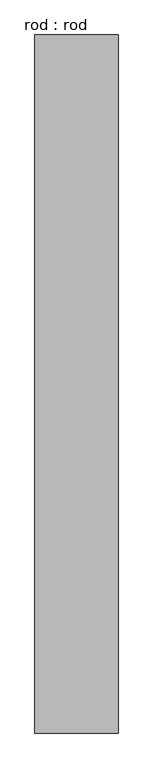
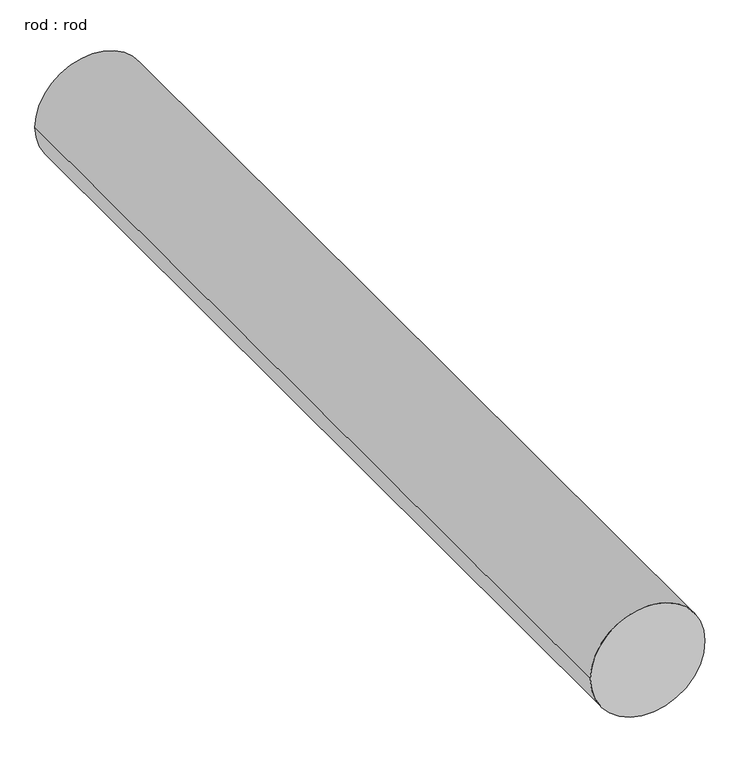
"""IFC4 building model written with IfcOpenShell, lengths in millimetres: proxy geometry, rod : rod."""

from ifc_helpers import new_model, si_unit, point, frame, frame_2d, origin, place, context, project, spatial, circle_curve, trimmed, segment, composite_curve, outline, extrude, source, transform, mapped, element, save


def rod_rod_80c61033(model_context):
    return source(origin(), model_context, "Body", "SweptSolid", [
        extrude(outline(composite_curve([segment(trimmed(circle_curve(frame_2d((0.0108462, 0.0)), 200.0), [point((0.0108462, 200.0))], [point((0.0108462, -200.0))], False, "CARTESIAN"), True, "CONTINUOUS"), segment(trimmed(circle_curve(frame_2d((0.0108462, 0.0)), 200.0), [point((0.0108462, -200.0))], [point((0.0108462, 200.0))], False, "CARTESIAN"), True, "CONTINUOUS")], self_intersect=False)), frame((0.0, 2412.7286153, 0.0), z_axis=(0.0, 1.0, 0.0), x_axis=(0.0, 0.0, 1.0)), (0.0, 0.0, 1.0), 3360.0),
    ])


if __name__ == "__main__":
    model = new_model("IFC4")
    model_context = context("Model", 3, world=origin())
    ifc_project = project(units=[si_unit("LENGTHUNIT", "METRE", prefix="MILLI")], contexts=[model_context])
    site = spatial("IfcSite", under=ifc_project)
    building = spatial("IfcBuilding", under=site)
    placement = place(None, origin())
    rod_rod_shape = rod_rod_80c61033(model_context)
    element("IfcBuildingElementProxy", 1, Name="rod : rod", ObjectType="rod : rod", at=placement, inside=building, context=model_context, shape_type="MappedRepresentation", body=[
        mapped(rod_rod_shape, transform((0.0, 0.0, 0.0), x_axis=(1.0, 0.0, 0.0), y_axis=(0.0, 1.0, 0.0), z_axis=(0.0, 0.0, 1.0))),
    ])
    save(model, "model.ifc")

# Revit data of these elements
# Type "rod : rod"
#   Default Elevation = 0
